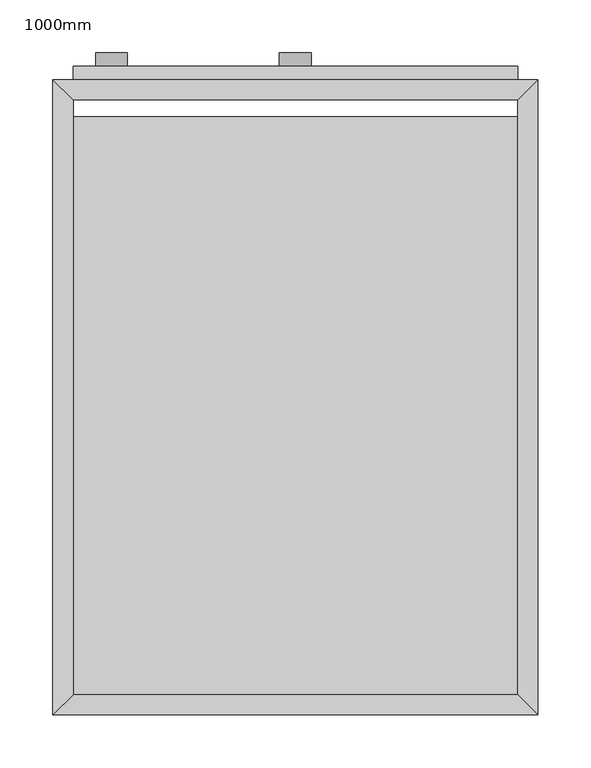
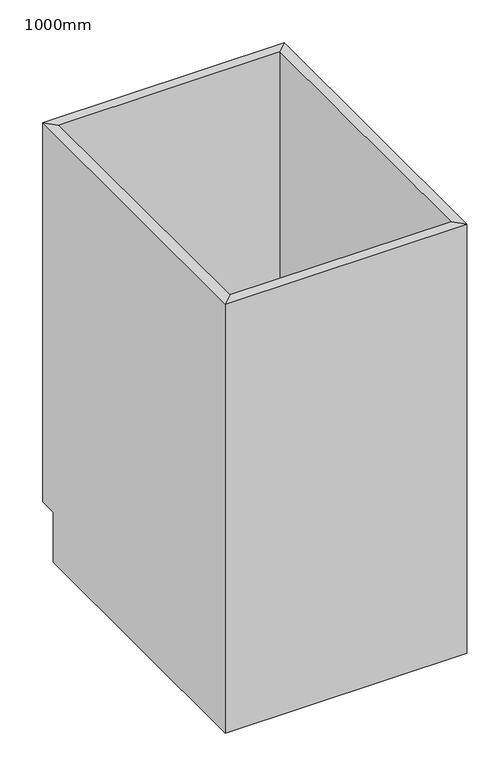
"""IFC4 building model written with IfcOpenShell, lengths in millimetres: furniture geometry, M_Base Cabinet-single &  Drawer-ROUND : 1000mm."""

from ifc_helpers import new_model, si_unit, point, frame, frame_2d, origin, place, context, project, spatial, polyline, circle_curve, trimmed, segment, composite_curve, outline, extrude, faceted_brep, source, transform, mapped, element, save


def furniture_1000mm_e0aacdb0(model_context):
    return source(origin(), model_context, "Body", "SolidModel", [
        faceted_brep([(507.6877049, 580.95, 860.0), (87.7877049, 580.95, 860.0), (87.7877049, 580.95, 100.0), (507.6877049, 580.95, 100.0), (526.7377049, 600.0, 860.0), (68.7377049, 600.0, 860.0), (526.7377049, 600.0, 100.0), (68.7377049, 600.0, 100.0), (87.7877049, 19.05, 860.0), (87.7877049, 19.05, 100.0), (87.7877049, 565.0, 100.0), (68.7377049, 0.0, 860.0), (68.7377049, 565.0, 100.0), (68.7377049, 565.0, 0.0), (68.7377049, 0.0, 0.0), (507.6877049, 19.05, 860.0), (507.6877049, 19.05, 100.0), (526.7377049, 0.0, 860.0), (526.7377049, 0.0, 0.0), (507.6877049, 565.0, 100.0), (526.7377049, 565.0, 0.0), (526.7377049, 565.0, 100.0)], [[[0, 1, 2, 3]], [[0, 4, 5, 1]], [[4, 6, 7, 5]], [[2, 7, 6, 3]], [[1, 8, 9, 10, 2]], [[5, 11, 8, 1]], [[7, 12, 13, 14, 11, 5]], [[2, 10, 12, 7]], [[8, 15, 16, 9]], [[11, 17, 15, 8]], [[11, 14, 18, 17]], [[3, 19, 16, 15, 0]], [[0, 15, 17, 4]], [[4, 17, 18, 20, 21, 6]], [[6, 21, 19, 3]], [[10, 9, 16, 19]], [[18, 14, 13, 20]], [[13, 12, 10, 19, 21, 20]]]),
        extrude(outline(composite_curve([segment(trimmed(circle_curve(frame_2d((809.2, 297.7377049)), 15.0), [point((809.2, 282.7377049))], [point((809.2, 312.7377049))], False, "CARTESIAN"), True, "CONTINUOUS"), segment(trimmed(circle_curve(frame_2d((809.2, 297.7377049)), 15.0), [point((809.2, 312.7377049))], [point((809.2, 282.7377049))], False, "CARTESIAN"), True, "CONTINUOUS")], self_intersect=False)), frame((0.0, 612.7, 0.0), z_axis=(0.0, 1.0, 0.0), x_axis=(0.0, 0.0, 1.0)), (0.0, 0.0, 1.0), 12.7),
        extrude(outline(composite_curve([segment(trimmed(circle_curve(frame_2d((631.4, 124.0127049)), 15.0), [point((631.4, 109.0127049))], [point((631.4, 139.0127049))], False, "CARTESIAN"), True, "CONTINUOUS"), segment(trimmed(circle_curve(frame_2d((631.4, 124.0127049)), 15.0), [point((631.4, 139.0127049))], [point((631.4, 109.0127049))], False, "CARTESIAN"), True, "CONTINUOUS")], self_intersect=False)), frame((0.0, 612.7, 0.0), z_axis=(0.0, 1.0, 0.0), x_axis=(0.0, 0.0, 1.0)), (0.0, 0.0, 1.0), 12.7),
        extrude(outline(polyline([(507.6877049, 612.7), (507.6877049, 600.0), (87.7877049, 600.0), (87.7877049, 612.7), (507.6877049, 612.7)])), frame((0.0, 0.0, 739.35), z_axis=(0.0, 0.0, 1.0), x_axis=(1.0, 0.0, 0.0)), (0.0, 0.0, 1.0), 101.6),
        extrude(outline(polyline([(507.6877049, 612.7), (507.6877049, 600.0), (87.7877049, 600.0), (87.7877049, 612.7), (507.6877049, 612.7)])), frame((0.0, 0.0, 119.05), z_axis=(0.0, 0.0, 1.0), x_axis=(1.0, 0.0, 0.0)), (0.0, 0.0, 1.0), 601.25),
    ])


if __name__ == "__main__":
    model = new_model("IFC4")
    model_context = context("Model", 3, world=origin())
    ifc_project = project(units=[si_unit("LENGTHUNIT", "METRE", prefix="MILLI")], contexts=[model_context])
    site = spatial("IfcSite", under=ifc_project)
    building = spatial("IfcBuilding", under=site)
    placement = place(None, origin())
    furniture_1000mm_shape = furniture_1000mm_e0aacdb0(model_context)
    element("IfcFurniture", 1, ObjectType="M_Base Cabinet-single &  Drawer-ROUND : 1000mm", at=placement, inside=building, context=model_context, shape_type="MappedRepresentation", body=[
        mapped(furniture_1000mm_shape, transform((0.0, 0.0, 0.0), x_axis=(1.0, 0.0, 0.0), y_axis=(0.0, 1.0, 0.0), z_axis=(0.0, 0.0, 1.0))),
    ])
    save(model, "model.ifc")

# Revit data of these elements
# Type "M_Base Cabinet-single &  Drawer-ROUND : 1000mm"
#   Depth = 1' - 11.62205"
#   Height = 2' - 9.85827"
#   Plinth Depth = 0' - 1.37795"
#   Plinth Height = 0' - 3.93701"
#   Width = 3' - 4"
#   Cabinet Material = Base cabinet 2120100 Aspekt - 83012120100 - White
#   Door/Drawer Material = Base cabinet 2120100 Aspekt - 83012120100 - White
#   Handle Material = Cabinets - Handles
#   Default Elevation = 0
# Element 1 (IfcFurniture, "M_Base Cabinet-single &  Drawer-ROUND : 1000mm")
#   Materials on its faces: "Base cabinet 2120100 Aspekt - 83012120100 - White", "Cabinets - Handles"
# Materials
#   "Base cabinet 2120100 Aspekt - 83012120100 - White": class "Miscellaneous", colour RGB 255 255 255, transparency 0, Manufacturer = "Marbodal", URL = "http://www.marbodal.se", Cost = 0
#   "Cabinets - Handles": class "Metal", colour RGB 57 57 57, transparency 0
